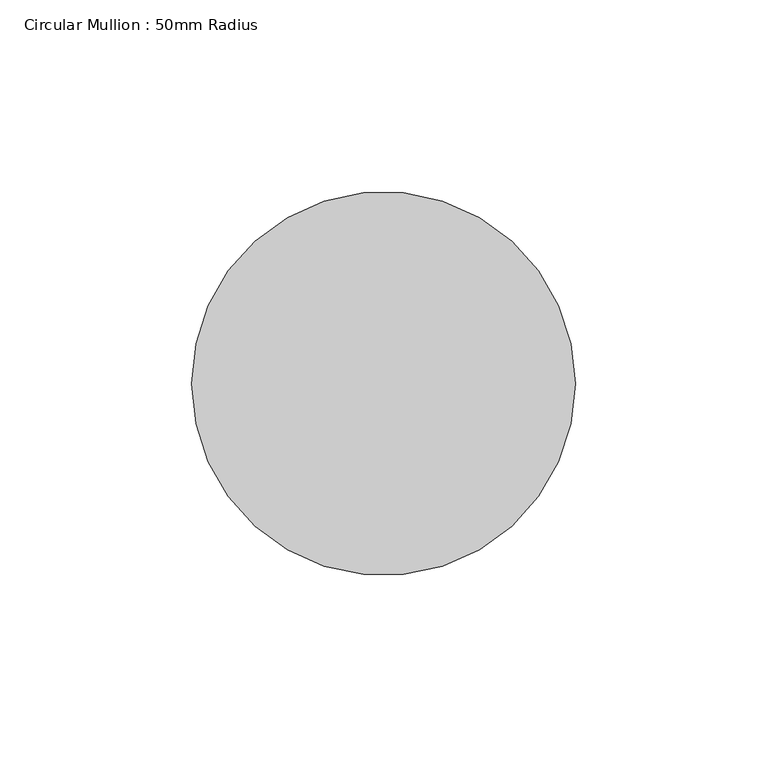
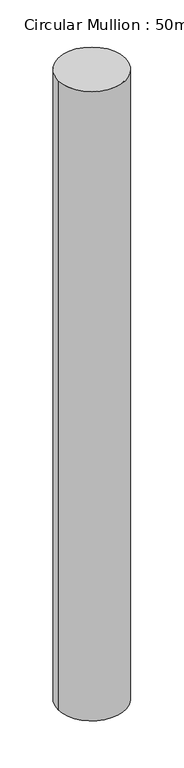
"""IFC4 building model written with IfcOpenShell, lengths in millimetres: member geometry, Circular Mullion : 50mm Radius."""

from ifc_helpers import new_model, si_unit, point, frame, origin, origin_2d, place, context, project, spatial, circle_curve, trimmed, segment, composite_curve, outline, extrude, source, transform, mapped, element, save


def circular_mullion_50mm_radius_3e48a9d2(model_context):
    return source(origin(), model_context, "Body", "SweptSolid", [
        extrude(outline(composite_curve([segment(trimmed(circle_curve(origin_2d(), 50.0), [point((50.0, 0.0))], [point((-50.0, 0.0))], False, "CARTESIAN"), True, "CONTINUOUS"), segment(trimmed(circle_curve(origin_2d(), 50.0), [point((-50.0, 0.0))], [point((50.0, 0.0))], False, "CARTESIAN"), True, "CONTINUOUS")], self_intersect=False)), frame((0.0, 0.0, -987.784473), z_axis=(0.0, 0.0, 1.0), x_axis=(1.0, 0.0, 0.0)), (0.0, 0.0, 1.0), 987.784473),
    ])


if __name__ == "__main__":
    model = new_model("IFC4")
    model_context = context("Model", 3, world=origin())
    ifc_project = project(units=[si_unit("LENGTHUNIT", "METRE", prefix="MILLI")], contexts=[model_context])
    site = spatial("IfcSite", under=ifc_project)
    building = spatial("IfcBuilding", under=site)
    placement = place(None, origin())
    circular_mullion_50mm_radius_shape = circular_mullion_50mm_radius_3e48a9d2(model_context)
    element("IfcMember", 1, ObjectType="Circular Mullion : 50mm Radius", at=placement, inside=building, context=model_context, shape_type="MappedRepresentation", body=[
        mapped(circular_mullion_50mm_radius_shape, transform((0.0, 0.0, 0.0), x_axis=(1.0, 0.0, 0.0), y_axis=(0.0, 1.0, 0.0), z_axis=(0.0, 0.0, 1.0))),
    ])
    save(model, "model.ifc")

# Revit data of these elements
# Type "Circular Mullion : 50mm Radius"
#   built-in parameter 1007350 = 0.164042 (stored number, unit not read)
# Element 1 (IfcMember, "Circular Mullion : 50mm Radius")
#   Materials on its faces: "Aluminium"
# Materials
#   "Aluminium": class "Metal", colour RGB 247 247 247, transparency 0, Description = "Aluminium 6061", Cost = 0
